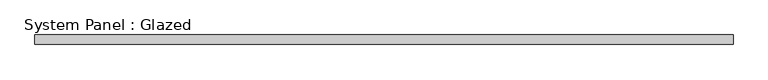
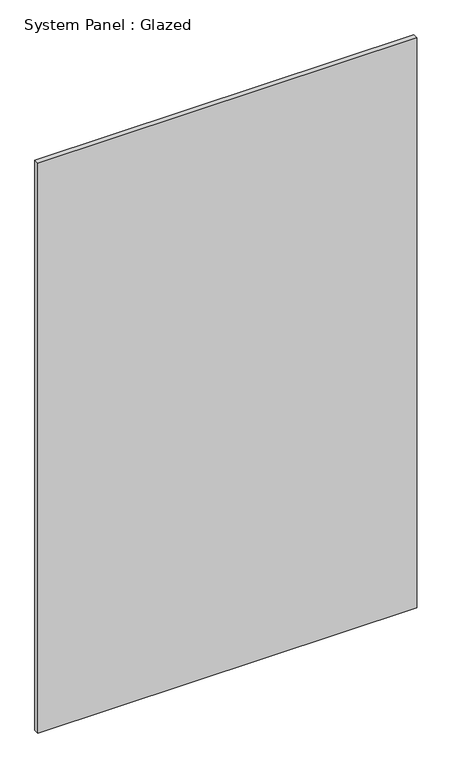
"""IFC4 building model written with IfcOpenShell, lengths in millimetres: plate geometry, System Panel : Glazed."""

from ifc_helpers import new_model, si_unit, origin, origin_with_axes, place, context, project, spatial, polyline, outline, extrude, source, transform, mapped, element, save


def system_panel_glazed_4d026453(model_context):
    return source(origin(), model_context, "Body", "SweptSolid", [
        extrude(outline(polyline([(919.4444444, 24.5), (-919.4444444, 24.5), (-919.4444444, 49.5), (919.4444444, 49.5), (919.4444444, 24.5)])), origin_with_axes(), (0.0, 0.0, 1.0), 2925.0),
    ])


if __name__ == "__main__":
    model = new_model("IFC4")
    model_context = context("Model", 3, world=origin())
    ifc_project = project(units=[si_unit("LENGTHUNIT", "METRE", prefix="MILLI")], contexts=[model_context])
    site = spatial("IfcSite", under=ifc_project)
    building = spatial("IfcBuilding", under=site)
    placement = place(None, origin())
    system_panel_glazed_shape = system_panel_glazed_4d026453(model_context)
    element("IfcPlate", 1, ObjectType="System Panel : Glazed", at=placement, inside=building, context=model_context, shape_type="MappedRepresentation", body=[
        mapped(system_panel_glazed_shape, transform((0.0, 0.0, 0.0), x_axis=(1.0, 0.0, 0.0), y_axis=(0.0, 1.0, 0.0), z_axis=(0.0, 0.0, 1.0))),
    ])
    save(model, "model.ifc")

# Revit data of these elements
# Element 1 (IfcPlate, "System Panel : Glazed")
#   Materials on its faces: "Glass"
# Materials
#   "Glass": class "Glass", colour RGB 0 128 192, transparency 0.9
